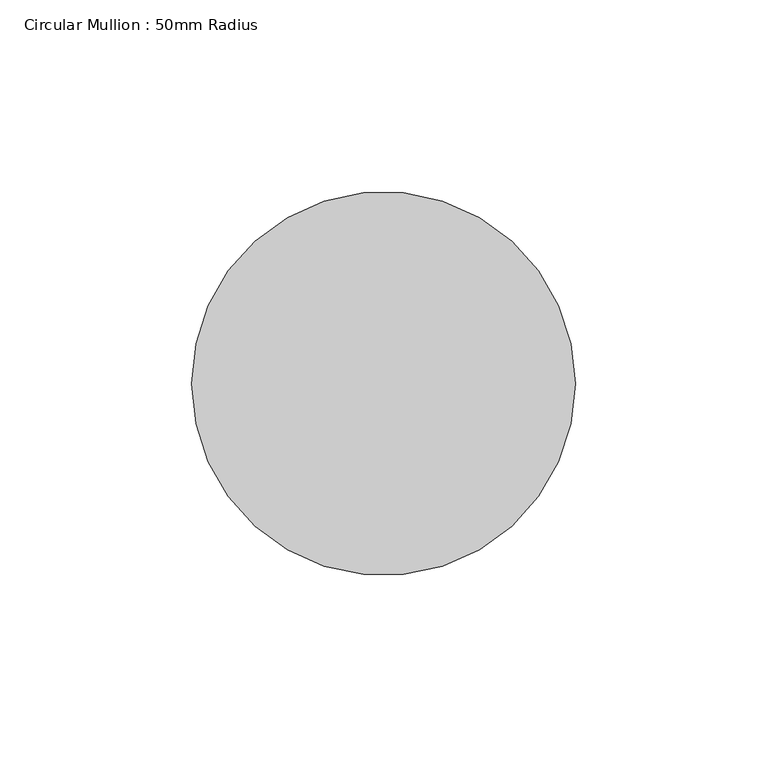
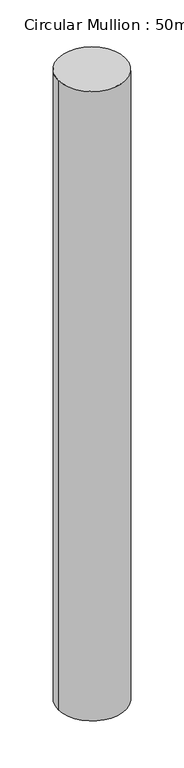
"""IFC4 building model written with IfcOpenShell, lengths in millimetres: member geometry, Circular Mullion : 50mm Radius."""

from ifc_helpers import new_model, si_unit, point, frame, origin, origin_2d, place, context, project, spatial, circle_curve, trimmed, segment, composite_curve, outline, extrude, source, transform, mapped, element, save


def circular_mullion_50mm_radius_10bcaec4(model_context):
    return source(origin(), model_context, "Body", "SweptSolid", [
        extrude(outline(composite_curve([segment(trimmed(circle_curve(origin_2d(), 50.0), [point((50.0, 0.0))], [point((-50.0, 0.0))], False, "CARTESIAN"), True, "CONTINUOUS"), segment(trimmed(circle_curve(origin_2d(), 50.0), [point((-50.0, 0.0))], [point((50.0, 0.0))], False, "CARTESIAN"), True, "CONTINUOUS")], self_intersect=False)), frame((0.0, 0.0, -989.8190797), z_axis=(0.0, 0.0, 1.0), x_axis=(1.0, 0.0, 0.0)), (0.0, 0.0, 1.0), 989.8190797),
    ])


if __name__ == "__main__":
    model = new_model("IFC4")
    model_context = context("Model", 3, world=origin())
    ifc_project = project(units=[si_unit("LENGTHUNIT", "METRE", prefix="MILLI")], contexts=[model_context])
    site = spatial("IfcSite", under=ifc_project)
    building = spatial("IfcBuilding", under=site)
    placement = place(None, origin())
    circular_mullion_50mm_radius_shape = circular_mullion_50mm_radius_10bcaec4(model_context)
    element("IfcMember", 1, ObjectType="Circular Mullion : 50mm Radius", at=placement, inside=building, context=model_context, shape_type="MappedRepresentation", body=[
        mapped(circular_mullion_50mm_radius_shape, transform((0.0, 0.0, 0.0), x_axis=(1.0, 0.0, 0.0), y_axis=(0.0, 1.0, 0.0), z_axis=(0.0, 0.0, 1.0))),
    ])
    save(model, "model.ifc")

# Revit data of these elements
# Type "Circular Mullion : 50mm Radius"
#   built-in parameter 1007350 = 0.164042 (stored number, unit not read)
# Element 1 (IfcMember, "Circular Mullion : 50mm Radius")
#   Materials on its faces: "Aluminium"
# Materials
#   "Aluminium": class "Metal", colour RGB 247 247 247, transparency 0, Description = "Aluminium 6061", Cost = 0
